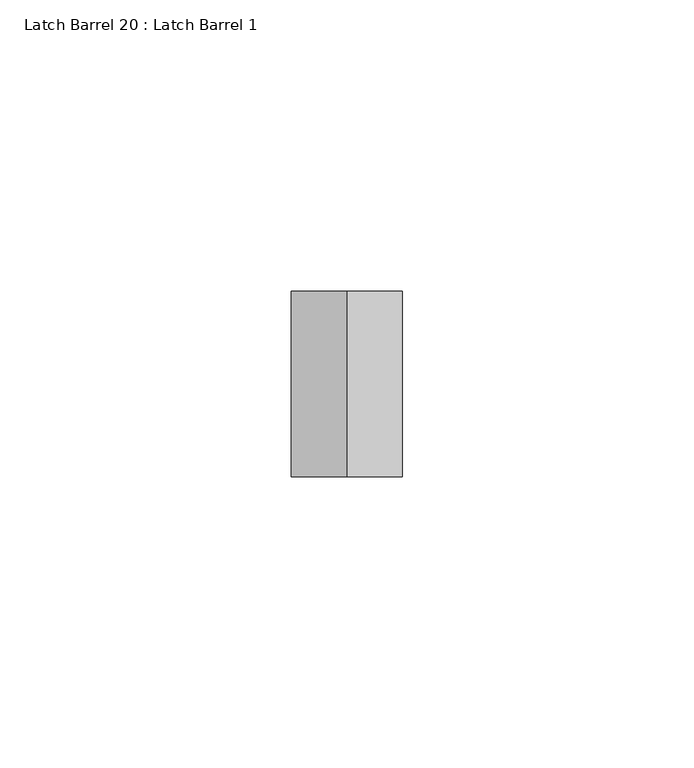
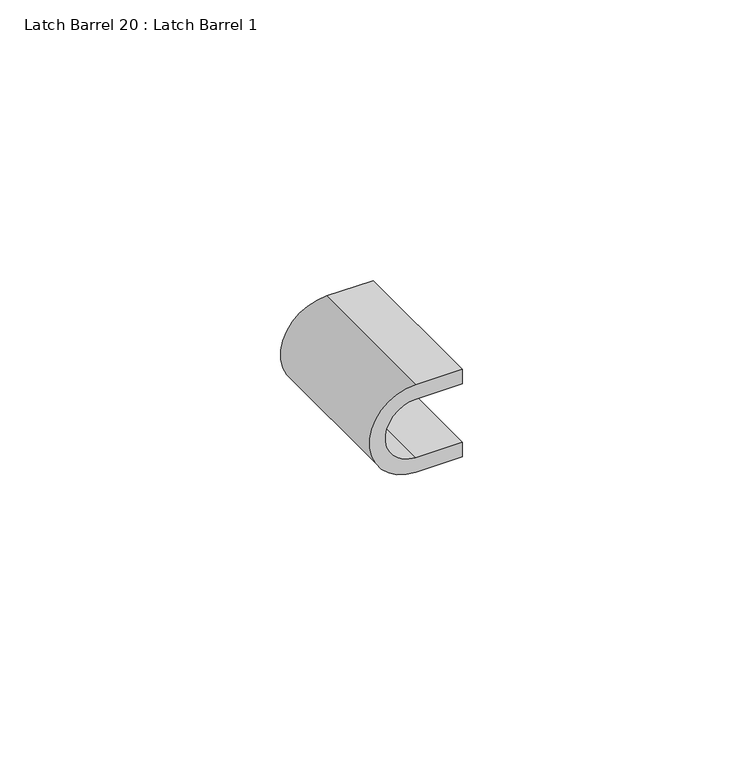
"""IFC4 building model written with IfcOpenShell, lengths in millimetres: proxy geometry, Latch Barrel 20 : Latch Barrel 1."""

from ifc_helpers import new_model, si_unit, point, frame, frame_2d, origin, place, context, project, spatial, polyline, circle_curve, trimmed, segment, composite_curve, outline, extrude, source, transform, mapped, element, save


def latch_barrel_20_latch_barrel_1_0ede4d69(model_context):
    return source(origin(), model_context, "Body", "SweptSolid", [
        extrude(outline(composite_curve([segment(trimmed(circle_curve(frame_2d((1066.8, 587312.7185739)), 6.35), [point((1060.45, 587312.7185739))], [point((1073.15, 587312.7185739))], True, "CARTESIAN"), True, "CONTINUOUS"), segment(polyline([(1073.15, 587312.7185739), (1073.15, 587322.2435739), (1076.325, 587322.2435739), (1076.325, 587312.7185739)]), True, "CONTINUOUS"), segment(trimmed(circle_curve(frame_2d((1066.8, 587312.7185739)), 9.525), [point((1076.325, 587312.7185739))], [point((1057.275, 587312.7185739))], False, "CARTESIAN"), True, "CONTINUOUS"), segment(polyline([(1057.275, 587312.7185739), (1057.275, 587322.2435739), (1060.45, 587322.2435739), (1060.45, 587312.7185739)]), True, "CONTINUOUS")], self_intersect=False)), frame((0.0, -535163.4663841, 0.0), z_axis=(0.0, 1.0, 0.0), x_axis=(0.0, 0.0, 1.0)), (0.0, 0.0, 1.0), 31.75),
    ])


if __name__ == "__main__":
    model = new_model("IFC4")
    model_context = context("Model", 3, world=origin())
    ifc_project = project(units=[si_unit("LENGTHUNIT", "METRE", prefix="MILLI")], contexts=[model_context])
    site = spatial("IfcSite", under=ifc_project)
    building = spatial("IfcBuilding", under=site)
    placement = place(None, origin())
    latch_barrel_20_latch_barrel_1_shape = latch_barrel_20_latch_barrel_1_0ede4d69(model_context)
    element("IfcBuildingElementProxy", 1, Name="Latch Barrel 20 : Latch Barrel 1", ObjectType="Latch Barrel 20 : Latch Barrel 1", at=placement, inside=building, context=model_context, shape_type="MappedRepresentation", body=[
        mapped(latch_barrel_20_latch_barrel_1_shape, transform((0.0, 0.0, 0.0), x_axis=(1.0, 0.0, 0.0), y_axis=(0.0, 1.0, 0.0), z_axis=(0.0, 0.0, 1.0))),
    ])
    save(model, "model.ifc")

# Revit data of these elements
# Element 1 (IfcBuildingElementProxy, "Latch Barrel 20 : Latch Barrel 1")
#   Materials on its faces: "GALV. GATE LATCH"
# Materials
#   "GALV. GATE LATCH": class "Metal", colour RGB 189 187 185, transparency 0, Description = "Carbon steel", Cost = 0
